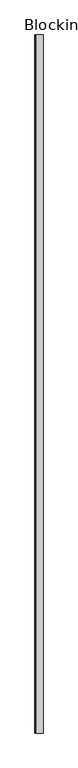
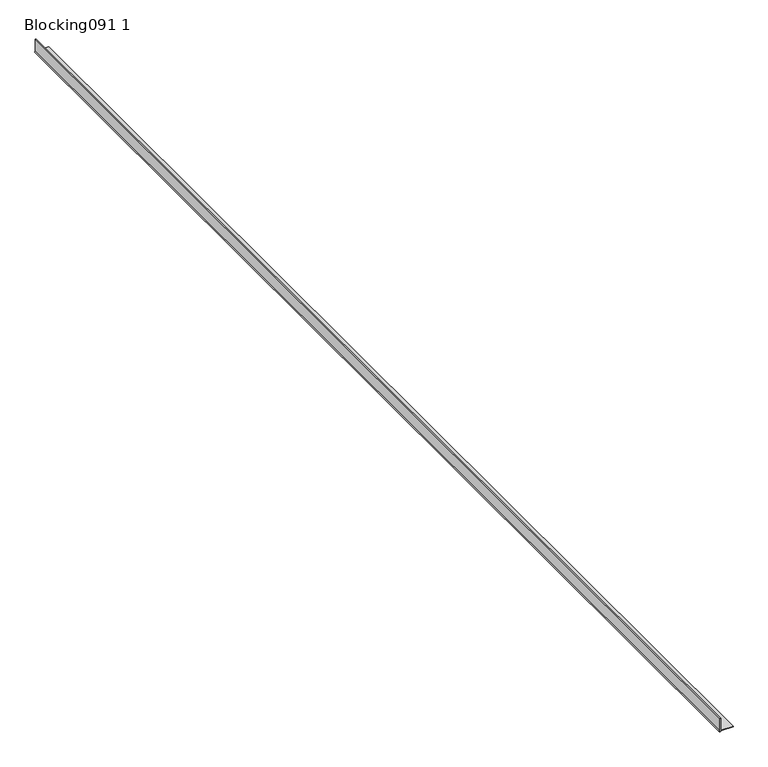
"""IFC4 building model written with IfcOpenShell, lengths in millimetres: proxy geometry, Blocking091 1 : Blocking091 17871."""

from ifc_helpers import new_model, si_unit, point, frame, frame_2d, origin, place, context, project, spatial, polyline, circle_curve, trimmed, segment, composite_curve, outline, extrude, source, transform, mapped, element, save


def blocking091_1_6a2c43f3(model_context):
    return source(origin(), model_context, "Body", "SweptSolid", [
        extrude(outline(composite_curve([segment(polyline([(39579.5041839, 7204.8513569), (39579.5041839, 7203.5713569), (39558.6202421, 7203.5713569)]), True, "CONTINUOUS"), segment(trimmed(circle_curve(frame_2d((39557.3733211, 7203.9204176)), 1.2948572), [point((39558.6202421, 7203.5713569))], [point((39557.071, 7205.1794876))], False, "CARTESIAN"), True, "CONTINUOUS"), segment(polyline([(39557.071, 7205.1794876), (39557.071, 7226.0045408), (39558.351, 7226.0045408), (39558.351, 7204.8513569), (39579.5041839, 7204.8513569)]), True, "CONTINUOUS")], self_intersect=False)), frame((0.0, -3747.9491938, 0.0), z_axis=(0.0, 1.0, 0.0), x_axis=(0.0, 0.0, 1.0)), (0.0, 0.0, 1.0), 2000.0),
    ])


if __name__ == "__main__":
    model = new_model("IFC4")
    model_context = context("Model", 3, world=origin())
    ifc_project = project(units=[si_unit("LENGTHUNIT", "METRE", prefix="MILLI")], contexts=[model_context])
    site = spatial("IfcSite", under=ifc_project)
    building = spatial("IfcBuilding", under=site)
    placement = place(None, origin())
    blocking091_1_shape = blocking091_1_6a2c43f3(model_context)
    element("IfcBuildingElementProxy", 1, Name="Blocking091 1 : Blocking091 17871", ObjectType="Blocking091 1 : Blocking091 17871", at=placement, inside=building, context=model_context, shape_type="MappedRepresentation", body=[
        mapped(blocking091_1_shape, transform((0.0, 0.0, 0.0), x_axis=(1.0, 0.0, 0.0), y_axis=(0.0, 1.0, 0.0), z_axis=(0.0, 0.0, 1.0))),
    ])
    save(model, "model.ifc")

# Revit data of these elements
# Type "Blocking091 1 : Blocking091 17871"
#   NameOverride = "Blocking091"
# Element 1 (IfcBuildingElementProxy, "Blocking091 1 : Blocking091 17871")
#   Materials on its faces: "CORNER BEAD"
# Materials
#   "CORNER BEAD": class "Unassigned", colour RGB 253 236 176, transparency 0, Cost = 0
